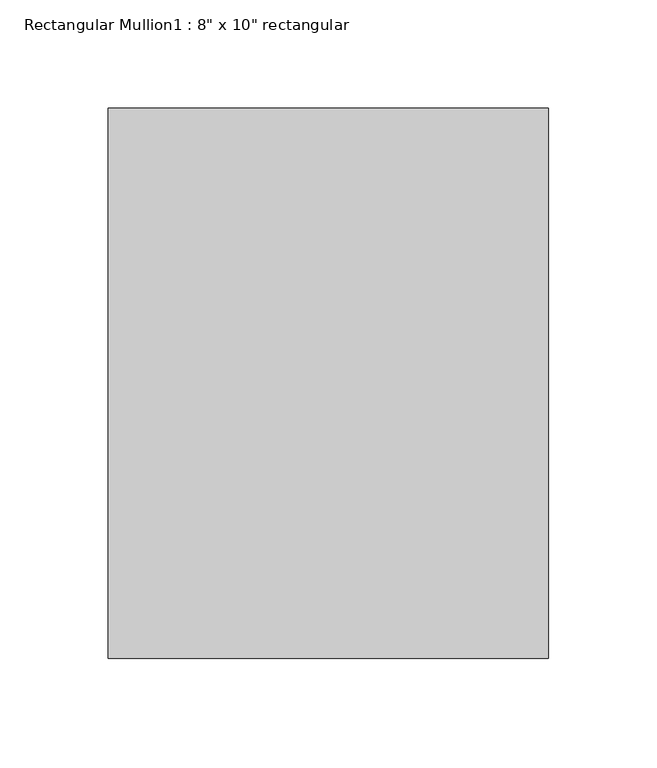
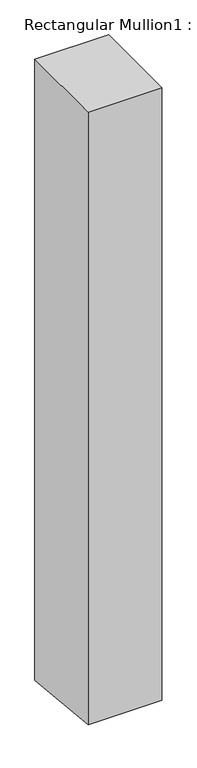
"""IFC4 building model written with IfcOpenShell, lengths in millimetres: member geometry."""

from ifc_helpers import new_model, si_unit, frame, origin, place, context, project, spatial, polyline, outline, extrude, source, transform, mapped, element, save


def member_7751821a(model_context):
    return source(origin(), model_context, "Body", "SweptSolid", [
        extrude(outline(polyline([(-127.0, 0.0), (127.0, 0.0), (127.0, -1809.0434772), (-127.0, -1785.0565228), (-127.0, 0.0)])), frame((-101.6, 0.0, 0.0), z_axis=(1.0, 0.0, 0.0), x_axis=(0.0, 1.0, 0.0)), (0.0, 0.0, 1.0), 203.2),
    ])


if __name__ == "__main__":
    model = new_model("IFC4")
    model_context = context("Model", 3, world=origin())
    ifc_project = project(units=[si_unit("LENGTHUNIT", "METRE", prefix="MILLI")], contexts=[model_context])
    site = spatial("IfcSite", under=ifc_project)
    building = spatial("IfcBuilding", under=site)
    placement = place(None, origin())
    member_shape = member_7751821a(model_context)
    element("IfcMember", 1, ObjectType="Rectangular Mullion1 : 8\" x 10\" rectangular", at=placement, inside=building, context=model_context, shape_type="MappedRepresentation", body=[
        mapped(member_shape, transform((0.0, 0.0, 0.0), x_axis=(1.0, 0.0, 0.0), y_axis=(0.0, 1.0, 0.0), z_axis=(0.0, 0.0, 1.0))),
    ])
    save(model, "model.ifc")

# Revit data of these elements
# Type "Rectangular Mullion1 : 8\" x 10\" rectangular"
#   built-in parameter 1007304 = 0.833333 (stored number, unit not read)
#   built-in parameter 1007301 = 0.333333 (stored number, unit not read)
#   built-in parameter 1007300 = 0.333333 (stored number, unit not read)
# Element 1 (IfcMember, "Rectangular Mullion1 : 8\" x 10\" rectangular")
#   Materials on its faces: "support-frame"
# Materials
#   "support-frame": class "Unassigned", colour RGB 233 233 233, transparency 0, Cost = 0
